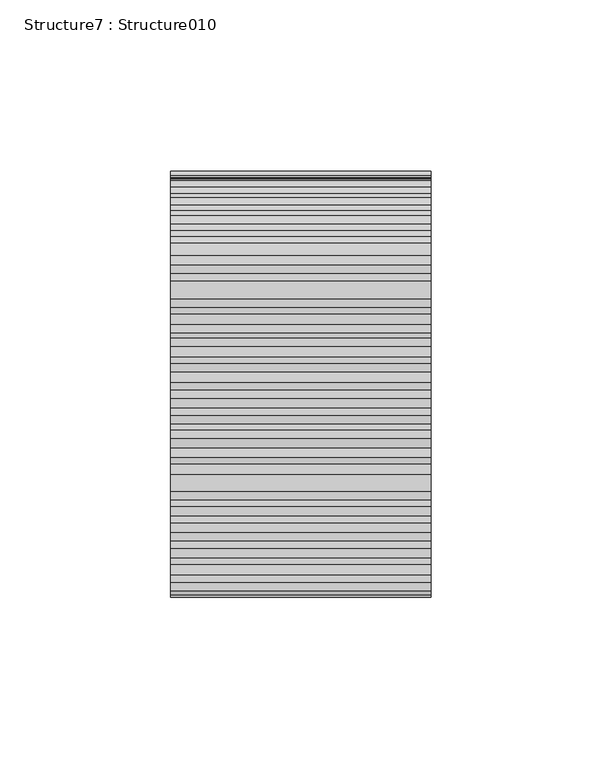
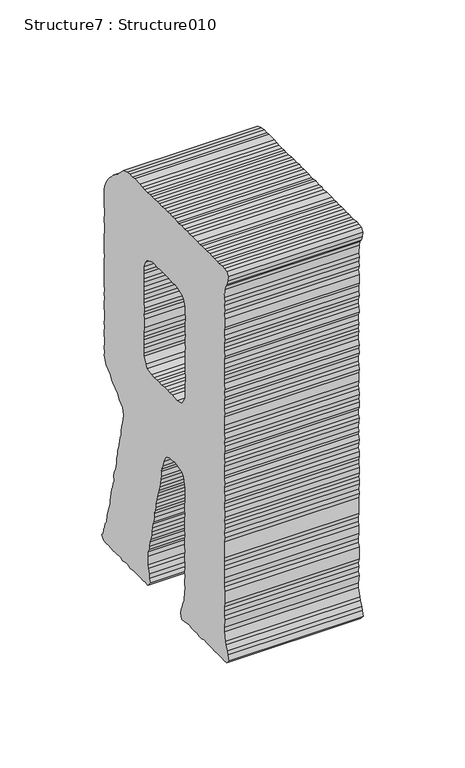
"""IFC4 building model written with IfcOpenShell, lengths in millimetres: proxy geometry, Structure7 : Structure010."""

from ifc_helpers import new_model, si_unit, frame, origin, place, context, project, spatial, polyline, outline, extrude, source, transform, mapped, element, save


def structure7_structure010_e7115294(model_context):
    return source(origin(), model_context, "Body", "SweptSolid", [
        extrude(outline(polyline([(1.8756485, -1e-07), (4.6342893, -0.4741019), (6.810177, -0.5377356), (9.8075758, -1.3631865), (11.9400118, -1.7296684), (14.0194728, -2.4093961), (17.1742837, -2.318918), (18.9568452, -2.9355861), (24.139316, -3.8262491), (26.9263797, -3.9949198), (29.3126025, -4.7153336), (31.4550578, -5.0835374), (33.8376019, -5.8153532), (36.6926695, -5.673361), (39.3323402, -6.7596827), (41.5102368, -6.8116273), (44.3215137, -6.9844594), (48.4740951, -8.3307909), (51.52246, -8.8546849), (53.762177, -8.6069382), (56.3918285, -9.6915379), (58.6449045, -9.446087), (61.3810019, -9.9163146), (63.1047438, -10.8452241), (65.5427678, -11.2642245), (68.6967438, -11.1736029), (71.0375061, -12.208554), (73.276388, -11.9606637), (77.4802226, -14.8794171), (78.3408152, -17.2244581), (79.8987954, -19.0678615), (82.0881858, -21.0086047), (83.5383892, -23.4541171), (84.1965, -25.1316935), (85.6488692, -27.5896125), (87.7822836, -29.8310514), (89.3402639, -31.6744548), (90.306611, -33.4041454), (94.0657227, -35.3043461), (99.1536322, -34.9246004), (102.2964149, -34.8440896), (104.536132, -34.5963428), (107.2855885, -35.0688663), (109.5762715, -34.5195628), (111.8159886, -34.2718161), (114.6172461, -34.4429263), (116.8947137, -33.890492), (119.1457808, -33.6567303), (121.6297613, -33.7733131), (124.1817458, -33.5792328), (127.2209263, -34.1015484), (131.7128844, -33.6082073), (134.3544206, -32.8080263), (137.1991298, -32.6762884), (139.8897666, -33.4610533), (141.8710262, -32.8465377), (144.6722838, -33.0176478), (146.7116849, -32.1148431), (149.505767, -32.2726857), (151.7519679, -32.0372281), (154.5916676, -31.9046292), (156.7249385, -32.2712546), (159.2810977, -32.0778918), (162.2264084, -31.3307773), (165.0681169, -31.1864892), (169.8053169, -31.0567862), (171.8488927, -30.1546989), (174.3855092, -29.9700119), (176.3792928, -29.3576487), (179.2283203, -29.2257932), (180.9596286, -28.2700395), (183.078849, -30.509039), (182.9715161, -33.0092223), (182.3434458, -34.788105), (182.2381218, -37.2765992), (181.7657418, -40.0252207), (181.0340694, -42.4069299), (180.2488741, -46.97572), (180.4984342, -49.2148891), (179.3560587, -52.1707149), (179.0430998, -53.9917185), (179.2408589, -56.5323008), (178.4135947, -59.5302474), (177.2078205, -66.5462459), (177.1442782, -68.731605), (176.1613237, -70.7598128), (176.3589393, -73.30123), (172.890139, -75.2237093), (170.9142802, -73.9411551), (168.5288923, -73.2208849), (165.8842119, -72.1337023), (164.1604701, -71.2047928), (159.2902667, -70.3677964), (156.5408102, -69.8952729), (154.196317, -70.7576788), (152.0112451, -70.6924666), (149.2233465, -70.5236523), (146.8666683, -71.3719296), (144.0248163, -71.5170526), (141.5358262, -71.3996089), (139.0384866, -71.2807302), (136.5516624, -71.1756931), (134.1958191, -72.024114), (131.4079206, -71.8552996), (128.9169216, -71.7495451), (126.3150014, -72.2341844), (124.0894784, -72.4843704), (121.9420134, -72.1153056), (119.1023138, -72.2479046), (116.5603487, -72.4437068), (113.9565631, -72.9392002), (112.0319574, -73.2290678), (109.1249453, -73.6733082), (106.9390383, -73.6079525), (104.0889805, -73.7508057), (101.8492634, -73.9985524), (98.7967238, -73.4739409), (96.8701092, -73.7754976), (94.2683326, -74.2593019), (91.1142131, -74.3507584), (86.7791193, -75.8020057), (84.6322417, -79.2058288), (84.1100696, -82.2441745), (83.1924188, -83.97243), (83.2710642, -87.126067), (83.755847, -91.6028006), (85.324877, -93.4369281), (88.8320152, -94.9826491), (91.4625016, -96.0673923), (98.4701507, -97.2717316), (101.0221351, -97.0776514), (104.0705, -97.6015454), (106.4020779, -98.634918), (108.8994175, -98.7537967), (110.774231, -98.7536532), (113.1534353, -99.4848951), (116.2151593, -100.0110851), (118.2882797, -100.6776887), (121.1391727, -100.5349791), (123.5897207, -100.9561319), (125.3569143, -101.5821933), (127.7506516, -102.3038984), (130.9054625, -102.2134203), (133.3418166, -102.6321338), (135.3703114, -103.6134183), (137.5035824, -103.9800437), (140.3544753, -103.837334), (142.9891363, -104.9227947), (145.4739517, -105.039521), (147.3083143, -105.3547758), (150.001795, -106.127995), (152.2314927, -105.8785263), (157.8298331, -106.2200293), (159.8236168, -105.6076661), (162.9745534, -105.5397314), (165.0067791, -104.6236591), (167.8618466, -104.4816669), (170.6989894, -106.2345921), (169.8717252, -109.2325389), (168.8411445, -111.5628775), (168.4745191, -113.6961484), (168.4066585, -115.8816249), (168.2475245, -118.6832215), (167.5158521, -121.0649307), (167.4621856, -123.2528466), (167.0417502, -125.69922), (166.0649795, -127.7164561), (165.9434524, -130.2142001), (165.0545114, -135.3866516), (164.9471784, -137.886835), (164.2673071, -139.967131), (163.3765007, -145.1504367), (163.3228342, -147.3383527), (162.9562088, -149.4716236), (159.8441581, -151.1339235), (157.2521138, -149.7454711), (155.2309379, -148.7766193), (152.6948693, -147.0874713), (150.9661178, -146.1577008), (146.2987873, -144.0902381), (143.8615982, -143.6713812), (138.8732596, -143.446748), (136.8589589, -142.4679028), (133.7517743, -142.2562502), (131.6631289, -141.574944), (129.1203289, -141.7706027), (122.1034955, -140.5646849), (119.7769271, -139.5321733), (117.3397381, -139.1133163), (114.2233692, -138.9000853), (109.6662683, -138.1168988), (107.2745398, -137.3835045), (104.8415255, -136.965365), (102.3505265, -136.8596105), (92.9015137, -135.2356968), (90.4125236, -135.118253), (88.0187862, -134.3965479), (84.9136106, -134.1732061), (82.4814313, -133.7552101), (80.6980348, -133.1383986), (78.2140544, -133.0218158), (75.1514955, -132.4954824), (72.7661075, -131.7752122), (70.6461956, -131.4108827), (68.4477644, -131.3433746), (65.711667, -130.873147), (63.6748228, -129.8904276), (60.8799057, -129.7324415), (58.3959252, -129.6158587), (55.7654389, -128.5311155), (53.868082, -128.5273847), (51.484703, -127.7954253), (48.3825281, -127.5846337), (45.8943729, -127.4673334), (44.1689612, -126.538137), (41.1164216, -126.0135254), (39.188972, -126.3149387), (36.4303312, -125.8408368), (34.3622203, -125.1750941), (31.8740652, -125.0577938), (28.8633074, -124.2300472), (27.0961138, -123.6039858), (24.3062064, -123.4468607), (19.1103765, -122.5539019), (17.2292225, -122.5409212), (14.5440912, -121.769137), (12.4654651, -121.0895526), (9.7143388, -120.6167422), (7.4762917, -120.8647759), (4.7911604, -120.0929917), (2.5935642, -120.0256271), (-0.3408402, -118.8886523), (-2.7872136, -118.4682169), (-5.273203, -118.3633233), (-7.0412314, -117.7371185), (-9.5447546, -117.6292116), (-11.9239589, -116.8979697), (-14.9731587, -116.3739321), (-16.9131324, -116.673193), (-19.9096962, -115.8478857), (-21.6910837, -115.219385), (-24.1224281, -114.8015325), (-26.6660632, -114.9970477), (-29.0598006, -114.2753426), (-32.1081655, -113.7514485), (-33.994329, -113.7376069), (-38.8636975, -112.900754), (-41.5075429, -111.8137149), (-44.0461683, -112.010091), (-46.7304647, -111.2384502), (-49.2336488, -111.1185671), (-51.3151187, -110.4505285), (-56.6023656, -110.1745246), (-59.1431568, -110.3584941), (-61.1845668, -111.2729881), (-63.7773026, -111.7592057), (-66.5743855, -111.588813), (-68.8175857, -109.9611723), (-68.6960587, -107.4634283), (-68.3292898, -105.3293224), (-67.5062004, -102.3306582), (-67.1913761, -100.4988005), (-67.0199134, -97.7104975), (-66.3523707, -95.6169079), (-66.2327091, -93.1300181), (-65.7623381, -90.3930858), (-65.0968043, -88.3111855), (-64.9233327, -85.5111932), (-64.3096, -83.7307061), (-64.1899384, -81.2438164), (-63.3509331, -76.3619238), (-62.5278436, -73.3632597), (-62.8158458, -71.4277997), (-61.7426482, -68.7944695), (-61.8751037, -65.953935), (-61.1506067, -63.5589582), (-60.536874, -61.7784711), (-60.7211305, -59.2393498), (-60.050587, -57.1583104), (-59.8841341, -54.3691464), (-59.1596371, -51.9741697), (-59.0969298, -49.7886672), (-57.9699222, -46.8422345), (-57.8483953, -44.3444906), (-57.5354364, -42.5234871), (-56.7123469, -39.5248228), (-56.2939204, -37.0901386), (-56.331671, -35.5191778), (-55.6123272, -33.1241749), (-55.0881462, -30.0741402), (-55.0740957, -28.2017661), (-54.9575784, -25.7031612), (-54.0666285, -20.5190205), (-53.396085, -18.437981), (-53.2814331, -15.9502303), (-52.2062266, -13.305211), (-50.3450419, -9.8531481), (-47.9105012, -8.396761), (-46.0652324, -6.8279266), (-43.6056435, -5.3758443), (-41.6671442, -3.1895068), (-40.1871179, -1.8802517), (-38.1039261, -0.6626226), (-35.8927754, 1.1545066), (-34.175661, 2.1126998), (-31.4143198, 3.5249571), (-27.1380456, 4.6639629), (-24.9509646, 4.6104399), (-20.0674022, 3.7711475), (-16.9764205, 3.5502452), (-15.1320387, 3.2332685), (-12.8012957, 2.2000394), (-10.3682814, 1.7818999), (-7.8254813, 1.9775586), (-2.436354, 0.4187135), (0.0, 0.0), (1.8756485, -1e-07)]), holes=[polyline([(45.0758029, -75.5357189), (45.9110774, -72.5511832), (45.9148082, -70.6538264), (46.4369804, -67.6154807), (47.5263808, -64.9729007), (47.6428981, -62.4742958), (47.955857, -60.6532923), (48.7839561, -57.655489), (48.5335611, -55.4161766), (48.7329678, -50.734678), (46.7410495, -49.4605385), (43.7545571, -46.7509985), (41.5703199, -46.6859298), (38.521955, -46.1620357), (36.7385586, -45.5452242), (33.9932768, -45.0734182), (31.8165542, -45.009641), (29.3852097, -44.5917885), (26.2708497, -44.3668682), (21.3964717, -43.5291543), (19.0027343, -42.8074492), (16.8168274, -42.7420935), (14.6835564, -42.3754681), (12.0510611, -41.3024142), (9.9177901, -40.9357887), (7.1165326, -40.7646785), (4.9824267, -40.3979096), (2.6012134, -39.6783569), (-0.2000442, -39.5072467), (-2.2815141, -38.8392081), (-5.0309706, -38.3666846), (-7.2168775, -38.3013289), (-9.2849884, -37.6355862), (-13.212562, -38.5362386), (-15.3598835, -40.0419872), (-17.9752667, -44.2962401), (-18.3936932, -46.7309243), (-18.0974851, -48.6686541), (-19.127231, -50.9991361), (-20.4384728, -58.6288152), (-20.6629105, -61.7303641), (-20.6664458, -63.6165798), (-21.6960482, -65.9462269), (-21.5034422, -68.4867832), (-20.7159155, -73.027581), (-19.8023479, -75.0593762), (-16.3545252, -76.9052189), (-14.2220891, -77.2717008), (-8.832127, -78.8306894), (-6.6024292, -78.5812207), (-1.4207934, -79.4717402), (0.3046183, -80.4009367), (3.1058759, -80.5720469), (5.2929569, -80.6255699), (8.2273613, -81.7625447), (10.1085153, -81.7755253), (19.5625377, -83.4003), (22.3607946, -83.55886), (24.3892894, -84.5401446), (26.8390025, -84.9611539), (29.627736, -85.1301118), (31.8156519, -85.1837782), (34.2611903, -85.6040701), (37.2465609, -86.4394882), (40.5587839, -85.4330812), (42.9674068, -84.2825557), (44.959429, -79.9091373), (45.0758029, -75.5357189)])]), frame((-35624.0862846, 278489.8631051, 4168.7393153), z_axis=(1.0, 0.0, 1.354250045437766e-12), x_axis=(1.3378719738997415e-12, 0.169377505791286, -0.9855512470348373)), (0.0, 0.0, 1.0), 76.2),
    ])


if __name__ == "__main__":
    model = new_model("IFC4")
    model_context = context("Model", 3, world=origin())
    ifc_project = project(units=[si_unit("LENGTHUNIT", "METRE", prefix="MILLI")], contexts=[model_context])
    site = spatial("IfcSite", under=ifc_project)
    building = spatial("IfcBuilding", under=site)
    placement = place(None, origin())
    structure7_structure010_shape = structure7_structure010_e7115294(model_context)
    element("IfcBuildingElementProxy", 1, Name="Structure7 : Structure010", ObjectType="Structure7 : Structure010", at=placement, inside=building, context=model_context, shape_type="MappedRepresentation", body=[
        mapped(structure7_structure010_shape, transform((0.0, 0.0, 0.0), x_axis=(1.0, 0.0, 0.0), y_axis=(0.0, 1.0, 0.0), z_axis=(0.0, 0.0, 1.0))),
    ])
    save(model, "model.ifc")

# Revit data of these elements
# Type "Structure7 : Structure010"
#   NameOverride = "Structure010"
# Element 1 (IfcBuildingElementProxy, "Structure7 : Structure010")
#   Materials on its faces: "BRUSHED ALUMINUM LETTERING"
# Materials
#   "BRUSHED ALUMINUM LETTERING": class "Unassigned", colour RGB 169 181 186, transparency 0, Cost = 0
